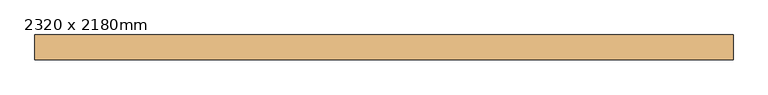
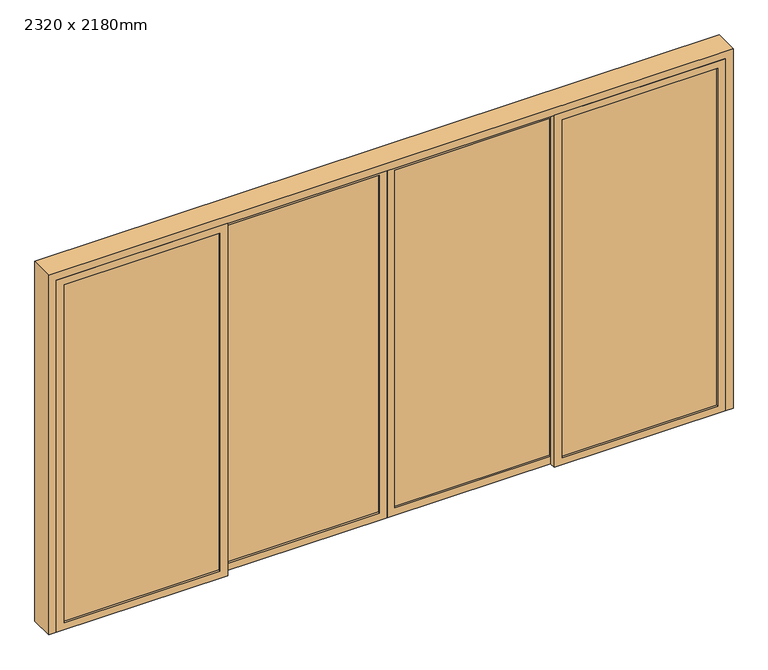
"""IFC4 building model written with IfcOpenShell, lengths in millimetres: door geometry, Porta envidraçada de correr quádrupla sem revestimento : 2320 x 2180mm."""

import ifcopenshell
import ifcopenshell.guid

model = None  # the IFC model being written
_history = None  # IfcOwnerHistory: only IFC2X3 demands one
_inside = {}  # id of a spatial element -> (the spatial element, [elements in it])
_under = {}  # id of a project, library or spatial element -> (it, [spatial elements below it])
_declared = {}  # id of a project -> (the project, [libraries it declares])
_typed = {}  # id of a type object -> (the type object, [elements of that type])
_made_of = {}  # id of a material, layer set ... -> (it, [elements and type objects made of it])


def new_model(schema):
    """Start an empty IFC model of exactly this schema.

    Asked for "IFC4X3", IfcOpenShell would pick the latest addendum, in which some entities
    have other attributes; the version numbers below select the first issue.
    IFC2X3 requires an IfcOwnerHistory on every rooted entity: one is made here for all.
    """
    global model, _history
    if schema == "IFC4X3":
        model = ifcopenshell.file(schema_version=(4, 3, 0, 0))
    else:
        model = ifcopenshell.file(schema=schema)
    _inside.clear()
    _under.clear()
    _declared.clear()
    _typed.clear()
    _made_of.clear()
    _history = None
    if model.schema == "IFC2X3":
        org = make("IfcOrganization", Name="unknown")
        user = make(
            "IfcPersonAndOrganization",
            ThePerson=make("IfcPerson", FamilyName="unknown"),
            TheOrganization=org,
        )
        app = make(
            "IfcApplication",
            ApplicationDeveloper=org,
            Version="unknown",
            ApplicationFullName="unknown",
            ApplicationIdentifier="unknown",
        )
        _history = make(
            "IfcOwnerHistory",
            OwningUser=user,
            OwningApplication=app,
            ChangeAction="ADDED",
            CreationDate=0,
        )
    return model


def make(cls, **values):
    """One entity of the class cls with the attributes given. An attribute that is None is left unset."""
    return model.create_entity(
        cls, **{name: value for name, value in values.items() if value is not None}
    )


def rooted(cls, **values):
    """An entity with a GlobalId (a new one), such as an element, a storey or a relation."""
    return make(cls, GlobalId=ifcopenshell.guid.new(), OwnerHistory=_history, **values)


def si_unit(unit_type, name, prefix=None):
    """IfcSIUnit, for example si_unit("LENGTHUNIT", "METRE", prefix="MILLI")."""
    return make("IfcSIUnit", UnitType=unit_type, Prefix=prefix, Name=name)


def assignment(units):
    """IfcUnitAssignment: the units of a project."""
    return None if units is None else make("IfcUnitAssignment", Units=units)


def point(xyz):
    """IfcCartesianPoint."""
    return None if xyz is None else make("IfcCartesianPoint", Coordinates=xyz)


def direction(xyz):
    """IfcDirection."""
    return None if xyz is None else make("IfcDirection", DirectionRatios=xyz)


def frame(location, z_axis=None, x_axis=None):
    """IfcAxis2Placement3D, a coordinate frame: its origin and axes. An axis left out is left unset."""
    return make(
        "IfcAxis2Placement3D",
        Location=point(location),
        Axis=direction(z_axis),
        RefDirection=direction(x_axis),
    )


def frame_2d(location, x_axis=None):
    """IfcAxis2Placement2D, a coordinate frame in the plane: its origin and x axis."""
    return make(
        "IfcAxis2Placement2D", Location=point(location), RefDirection=direction(x_axis)
    )


def origin():
    """The frame at (0, 0, 0) with its axes left unset."""
    return frame((0.0, 0.0, 0.0))


def place(relative_to, where):
    """IfcLocalPlacement: puts the frame where relative to a parent placement (None: the world)."""
    return make(
        "IfcLocalPlacement", PlacementRelTo=relative_to, RelativePlacement=where
    )


def context(
    kind, dimensions, precision=None, world=None, true_north=None, identifier=None
):
    """IfcGeometricRepresentationContext, for example the 3D "Model" context."""
    return make(
        "IfcGeometricRepresentationContext",
        ContextIdentifier=identifier,
        ContextType=kind,
        CoordinateSpaceDimension=dimensions,
        Precision=precision,
        WorldCoordinateSystem=world,
        TrueNorth=true_north,
    )


def project(units=None, contexts=None):
    """IfcProject with its units and contexts."""
    return rooted(
        "IfcProject",
        Name="project",
        RepresentationContexts=contexts,
        UnitsInContext=assignment(units),
    )


def spatial(cls, under=None, at=None, **own):
    """A site, building, storey or space (cls), placed at a placement, below another one or the project."""
    s = rooted(cls, ObjectPlacement=at, **own)
    if under is not None:
        _under.setdefault(under.id(), (under, []))[1].append(s)
    return s


def polyline(points):
    """IfcPolyline through the points."""
    return make("IfcPolyline", Points=[point(p) for p in points])


def circle_curve(where, radius):
    """IfcCircle in the frame where."""
    return make("IfcCircle", Position=where, Radius=radius)


def trimmed(basis, trim1, trim2, sense, master):
    """IfcTrimmedCurve: the piece of a basis curve between two trims."""
    return make(
        "IfcTrimmedCurve",
        BasisCurve=basis,
        Trim1=trim1,
        Trim2=trim2,
        SenseAgreement=sense,
        MasterRepresentation=master,
    )


def segment(curve, same_sense, transition):
    """IfcCompositeCurveSegment."""
    return make(
        "IfcCompositeCurveSegment",
        Transition=transition,
        SameSense=same_sense,
        ParentCurve=curve,
    )


def composite_curve(segments, self_intersect=None):
    """IfcCompositeCurve: segments joined end to end."""
    return make("IfcCompositeCurve", Segments=segments, SelfIntersect=self_intersect)


def outline(outer, holes=None, kind="AREA"):
    """IfcArbitraryClosedProfileDef: a profile drawn as a closed curve; with holes, ...WithVoids."""
    if holes is None:
        return make("IfcArbitraryClosedProfileDef", ProfileType=kind, OuterCurve=outer)
    return make(
        "IfcArbitraryProfileDefWithVoids",
        ProfileType=kind,
        OuterCurve=outer,
        InnerCurves=holes,
    )


def extrude(swept, where, along, depth):
    """IfcExtrudedAreaSolid: the profile swept, set in the frame where, extruded along a direction by depth."""
    return make(
        "IfcExtrudedAreaSolid",
        SweptArea=swept,
        Position=where,
        ExtrudedDirection=direction(along),
        Depth=depth,
    )


def shape(context_of_items, identifier, shape_type, items):
    """IfcShapeRepresentation: the items that make up one representation, for example the "Body"."""
    return make(
        "IfcShapeRepresentation",
        ContextOfItems=context_of_items,
        RepresentationIdentifier=identifier,
        RepresentationType=shape_type,
        Items=items,
    )


def source(mapping_origin, context_of_items, identifier, shape_type, items):
    """IfcRepresentationMap: a shape defined once, which mapped items show again and again."""
    return make(
        "IfcRepresentationMap",
        MappingOrigin=mapping_origin,
        MappedRepresentation=shape(context_of_items, identifier, shape_type, items),
    )


def transform(
    local_origin,
    x_axis=None,
    y_axis=None,
    z_axis=None,
    scale=None,
    scale2=None,
    scale3=None,
    uniform=True,
):
    """IfcCartesianTransformationOperator3D, or its non-uniform kind. x_axis, y_axis, z_axis: its Axis1, 2, 3."""
    if uniform:
        return make(
            "IfcCartesianTransformationOperator3D",
            Axis1=direction(x_axis),
            Axis2=direction(y_axis),
            LocalOrigin=point(local_origin),
            Scale=scale,
            Axis3=direction(z_axis),
        )
    return make(
        "IfcCartesianTransformationOperator3DnonUniform",
        Axis1=direction(x_axis),
        Axis2=direction(y_axis),
        LocalOrigin=point(local_origin),
        Scale=scale,
        Axis3=direction(z_axis),
        Scale2=scale2,
        Scale3=scale3,
    )


def mapped(mapping_source, mapping_target):
    """IfcMappedItem: shows the shape of a source again, moved by a transform."""
    return make(
        "IfcMappedItem", MappingSource=mapping_source, MappingTarget=mapping_target
    )


def made_of(thing, what):
    """Note that an element or type object is made of a material, layer set ...; save() writes the relation."""
    if what is not None:
        _made_of.setdefault(what.id(), (what, []))[1].append(thing)
    return thing


def element(
    cls,
    number,
    at=None,
    inside=None,
    cuts=None,
    type_object=None,
    material=None,
    context=None,
    identifier="Body",
    shape_type=None,
    held_by="IfcProductDefinitionShape",
    body=None,
    shapes=None,
    **own,
):
    """One element of the class cls, such as IfcWall. Its Tag is "e" and its number.

    at: its placement. inside: the storey or other place that contains it. cuts: it is an
    opening in that element (IfcRelVoidsElement). A single representation is given by context,
    identifier, shape_type and body (its items); several are given by shapes. held_by: the class
    of the entity that holds the representations. save() writes the other relations.
    """
    e = rooted(cls, Tag="e%d" % number, ObjectPlacement=at, **own)
    if body is not None:
        shapes = [shape(context, identifier, shape_type, body)]
    if shapes is not None:
        e.Representation = make(held_by, Representations=shapes)
    if inside is not None:
        _inside.setdefault(inside.id(), (inside, []))[1].append(e)
    if cuts is not None:
        rooted(
            "IfcRelVoidsElement", RelatingBuildingElement=cuts, RelatedOpeningElement=e
        )
    if type_object is not None:
        _typed.setdefault(type_object.id(), (type_object, []))[1].append(e)
    return made_of(e, material)


def aggregate(whole, parts):
    """IfcRelAggregates: a whole, such as a stair, and the parts it consists of."""
    return rooted("IfcRelAggregates", RelatingObject=whole, RelatedObjects=parts)


def save(model, path):
    """Write the relations noted so far, then the file.

    IfcRelAggregates (storeys below a building ...), IfcRelContainedInSpatialStructure (elements
    in a storey), IfcRelDefinesByType, IfcRelAssociatesMaterial and IfcRelDeclares: one each for
    every whole, place, type object, material and project.
    """
    for whole, parts in _under.values():
        aggregate(whole, parts)
    for where, things in _inside.values():
        rooted(
            "IfcRelContainedInSpatialStructure",
            RelatedElements=things,
            RelatingStructure=where,
        )
    for kind, things in _typed.values():
        rooted("IfcRelDefinesByType", RelatedObjects=things, RelatingType=kind)
    for what, things in _made_of.values():
        rooted("IfcRelAssociatesMaterial", RelatedObjects=things, RelatingMaterial=what)
    for by, libraries in _declared.values():
        rooted("IfcRelDeclares", RelatingContext=by, RelatedDefinitions=libraries)
    model.write(path)


def door_2320_x_2180mm_da102013(model_context):
    return source(origin(), model_context, "Body", "SweptSolid", [
        extrude(outline(composite_curve([segment(trimmed(circle_curve(frame_2d((990.0, 15.0)), 10.0), [point((1000.0, 15.0))], [point((990.0, 5.0))], False, "CARTESIAN"), True, "CONTINUOUS"), segment(polyline([(990.0, 5.0), (810.0, 5.0)]), True, "CONTINUOUS"), segment(trimmed(circle_curve(frame_2d((810.0, 15.0)), 10.0), [point((810.0, 5.0))], [point((800.0, 15.0))], False, "CARTESIAN"), True, "CONTINUOUS"), segment(polyline([(800.0, 15.0), (800.0, 35.0)]), True, "CONTINUOUS"), segment(trimmed(circle_curve(frame_2d((810.0, 35.0)), 10.0), [point((800.0, 35.0))], [point((810.0, 45.0))], False, "CARTESIAN"), True, "CONTINUOUS"), segment(polyline([(810.0, 45.0), (990.0, 45.0)]), True, "CONTINUOUS"), segment(trimmed(circle_curve(frame_2d((990.0, 35.0)), 10.0), [point((990.0, 45.0))], [point((1000.0, 35.0))], False, "CARTESIAN"), True, "CONTINUOUS"), segment(polyline([(1000.0, 35.0), (1000.0, 15.0)]), True, "CONTINUOUS")], self_intersect=False), holes=[composite_curve([segment(trimmed(circle_curve(frame_2d((985.0, 25.0)), 5.0), [point((985.0, 20.0))], [point((985.0, 30.0))], True, "CARTESIAN"), True, "CONTINUOUS"), segment(trimmed(circle_curve(frame_2d((985.0, 25.0)), 5.0), [point((985.0, 30.0))], [point((985.0, 20.0))], True, "CARTESIAN"), True, "CONTINUOUS")], self_intersect=False), composite_curve([segment(trimmed(circle_curve(frame_2d((815.0, 25.0)), 5.0), [point((815.0, 20.0))], [point((815.0, 30.0))], True, "CARTESIAN"), True, "CONTINUOUS"), segment(trimmed(circle_curve(frame_2d((815.0, 25.0)), 5.0), [point((815.0, 30.0))], [point((815.0, 20.0))], True, "CARTESIAN"), True, "CONTINUOUS")], self_intersect=False), composite_curve([segment(polyline([(960.0, 15.0), (960.0, 35.0)]), True, "CONTINUOUS"), segment(trimmed(circle_curve(frame_2d((955.0, 35.0)), 5.0), [point((960.0, 35.0))], [point((955.0, 40.0))], True, "CARTESIAN"), True, "CONTINUOUS"), segment(polyline([(955.0, 40.0), (845.0, 40.0)]), True, "CONTINUOUS"), segment(trimmed(circle_curve(frame_2d((845.0, 35.0)), 5.0), [point((845.0, 40.0))], [point((840.0, 35.0))], True, "CARTESIAN"), True, "CONTINUOUS"), segment(polyline([(840.0, 35.0), (840.0, 15.0)]), True, "CONTINUOUS"), segment(trimmed(circle_curve(frame_2d((845.0, 15.0)), 5.0), [point((840.0, 15.0))], [point((845.0, 10.0))], True, "CARTESIAN"), True, "CONTINUOUS"), segment(polyline([(845.0, 10.0), (955.0, 10.0)]), True, "CONTINUOUS"), segment(trimmed(circle_curve(frame_2d((955.0, 15.0)), 5.0), [point((955.0, 10.0))], [point((960.0, 15.0))], True, "CARTESIAN"), True, "CONTINUOUS")], self_intersect=False)]), frame((0.0, 5.4, 0.0), z_axis=(0.0, 1.0, 0.0), x_axis=(0.0, 0.0, 1.0)), (0.0, 0.0, 1.0), 3.0),
        extrude(outline(composite_curve([segment(trimmed(circle_curve(frame_2d((990.0, -35.0)), 10.0), [point((1000.0, -35.0))], [point((990.0, -45.0))], False, "CARTESIAN"), True, "CONTINUOUS"), segment(polyline([(990.0, -45.0), (810.0, -45.0)]), True, "CONTINUOUS"), segment(trimmed(circle_curve(frame_2d((810.0, -35.0)), 10.0), [point((810.0, -45.0))], [point((800.0, -35.0))], False, "CARTESIAN"), True, "CONTINUOUS"), segment(polyline([(800.0, -35.0), (800.0, -15.0)]), True, "CONTINUOUS"), segment(trimmed(circle_curve(frame_2d((810.0, -15.0)), 10.0), [point((800.0, -15.0))], [point((810.0, -5.0))], False, "CARTESIAN"), True, "CONTINUOUS"), segment(polyline([(810.0, -5.0), (990.0, -5.0)]), True, "CONTINUOUS"), segment(trimmed(circle_curve(frame_2d((990.0, -15.0)), 10.0), [point((990.0, -5.0))], [point((1000.0, -15.0))], False, "CARTESIAN"), True, "CONTINUOUS"), segment(polyline([(1000.0, -15.0), (1000.0, -35.0)]), True, "CONTINUOUS")], self_intersect=False), holes=[composite_curve([segment(trimmed(circle_curve(frame_2d((985.0, -25.0)), 5.0), [point((985.0, -30.0))], [point((985.0, -20.0))], True, "CARTESIAN"), True, "CONTINUOUS"), segment(trimmed(circle_curve(frame_2d((985.0, -25.0)), 5.0), [point((985.0, -20.0))], [point((985.0, -30.0))], True, "CARTESIAN"), True, "CONTINUOUS")], self_intersect=False), composite_curve([segment(trimmed(circle_curve(frame_2d((815.0, -25.0)), 5.0), [point((815.0, -30.0))], [point((815.0, -20.0))], True, "CARTESIAN"), True, "CONTINUOUS"), segment(trimmed(circle_curve(frame_2d((815.0, -25.0)), 5.0), [point((815.0, -20.0))], [point((815.0, -30.0))], True, "CARTESIAN"), True, "CONTINUOUS")], self_intersect=False), composite_curve([segment(polyline([(960.0, -35.0), (960.0, -15.0)]), True, "CONTINUOUS"), segment(trimmed(circle_curve(frame_2d((955.0, -15.0)), 5.0), [point((960.0, -15.0))], [point((955.0, -10.0))], True, "CARTESIAN"), True, "CONTINUOUS"), segment(polyline([(955.0, -10.0), (845.0, -10.0)]), True, "CONTINUOUS"), segment(trimmed(circle_curve(frame_2d((845.0, -15.0)), 5.0), [point((845.0, -10.0))], [point((840.0, -15.0))], True, "CARTESIAN"), True, "CONTINUOUS"), segment(polyline([(840.0, -15.0), (840.0, -35.0)]), True, "CONTINUOUS"), segment(trimmed(circle_curve(frame_2d((845.0, -35.0)), 5.0), [point((840.0, -35.0))], [point((845.0, -40.0))], True, "CARTESIAN"), True, "CONTINUOUS"), segment(polyline([(845.0, -40.0), (955.0, -40.0)]), True, "CONTINUOUS"), segment(trimmed(circle_curve(frame_2d((955.0, -35.0)), 5.0), [point((955.0, -40.0))], [point((960.0, -35.0))], True, "CARTESIAN"), True, "CONTINUOUS")], self_intersect=False)]), frame((0.0, 5.4, 0.0), z_axis=(0.0, 1.0, 0.0), x_axis=(0.0, 0.0, 1.0)), (0.0, 0.0, 1.0), 3.0),
        extrude(outline(polyline([(2450.0, -1125.0), (0.0, -1125.0), (0.0, 0.0), (2450.0, 0.0), (2450.0, -1125.0)]), holes=[polyline([(2400.0, -50.0), (50.0, -50.0), (50.0, -1075.0), (2400.0, -1075.0), (2400.0, -50.0)])]), frame((0.0, -34.6, 0.0), z_axis=(0.0, 1.0, 0.0), x_axis=(0.0, 0.0, 1.0)), (0.0, 0.0, 1.0), 40.0),
        extrude(outline(polyline([(2450.0, 1075.0), (0.0, 1075.0), (0.0, 2200.0), (2450.0, 2200.0), (2450.0, 1075.0)]), holes=[polyline([(2400.0, 2150.0), (50.0, 2150.0), (50.0, 1125.0), (2400.0, 1125.0), (2400.0, 2150.0)])]), frame((0.0, -79.6, 0.0), z_axis=(0.0, 1.0, 0.0), x_axis=(0.0, 0.0, 1.0)), (0.0, 0.0, 1.0), 40.0),
        extrude(outline(polyline([(2450.0, 0.0), (0.0, 0.0), (0.0, 1125.0), (2450.0, 1125.0), (2450.0, 0.0)]), holes=[polyline([(2400.0, 1075.0), (50.0, 1075.0), (50.0, 50.0), (2400.0, 50.0), (2400.0, 1075.0)])]), frame((0.0, -34.6, 0.0), z_axis=(0.0, 1.0, 0.0), x_axis=(0.0, 0.0, 1.0)), (0.0, 0.0, 1.0), 40.0),
        extrude(outline(polyline([(2450.0, -2200.0), (0.0, -2200.0), (0.0, -1075.0), (2450.0, -1075.0), (2450.0, -2200.0)]), holes=[polyline([(2400.0, -1125.0), (50.0, -1125.0), (50.0, -2150.0), (2400.0, -2150.0), (2400.0, -1125.0)])]), frame((0.0, -79.6, 0.0), z_axis=(0.0, 1.0, 0.0), x_axis=(0.0, 0.0, 1.0)), (0.0, 0.0, 1.0), 40.0),
        extrude(outline(polyline([(0.0, 2200.0), (0.0, 2250.0), (2500.0, 2250.0), (2500.0, -2250.0), (0.0, -2250.0), (0.0, -2200.0), (2450.0, -2200.0), (2450.0, 2200.0), (0.0, 2200.0)])), frame((0.0, -79.6, 0.0), z_axis=(0.0, 1.0, 0.0), x_axis=(0.0, 0.0, 1.0)), (0.0, 0.0, 1.0), 159.2),
        extrude(outline(polyline([(1075.0, -7.6), (1075.0, -21.6), (50.0, -21.6), (50.0, -7.6), (1075.0, -7.6)])), frame((0.0, 0.0, 50.0), z_axis=(0.0, 0.0, 1.0), x_axis=(1.0, 0.0, 0.0)), (0.0, 0.0, 1.0), 2350.0),
        extrude(outline(polyline([(2150.0, -52.6), (2150.0, -66.6), (1125.0, -66.6), (1125.0, -52.6), (2150.0, -52.6)])), frame((0.0, 0.0, 50.0), z_axis=(0.0, 0.0, 1.0), x_axis=(1.0, 0.0, 0.0)), (0.0, 0.0, 1.0), 2350.0),
        extrude(outline(polyline([(-1125.0, -52.6), (-1125.0, -66.6), (-2150.0, -66.6), (-2150.0, -52.6), (-1125.0, -52.6)])), frame((0.0, 0.0, 50.0), z_axis=(0.0, 0.0, 1.0), x_axis=(1.0, 0.0, 0.0)), (0.0, 0.0, 1.0), 2350.0),
        extrude(outline(polyline([(-50.0, -7.6), (-50.0, -21.6), (-1075.0, -21.6), (-1075.0, -7.6), (-50.0, -7.6)])), frame((0.0, 0.0, 50.0), z_axis=(0.0, 0.0, 1.0), x_axis=(1.0, 0.0, 0.0)), (0.0, 0.0, 1.0), 2350.0),
        extrude(outline(polyline([(-1125.0, -52.6), (-1125.0, -66.6), (-2150.0, -66.6), (-2150.0, -52.6), (-1125.0, -52.6)])), frame((0.0, 0.0, 50.0), z_axis=(0.0, 0.0, 1.0), x_axis=(1.0, 0.0, 0.0)), (0.0, 0.0, 1.0), 2350.0),
        extrude(outline(polyline([(-50.0, -7.6), (-50.0, -21.6), (-1075.0, -21.6), (-1075.0, -7.6), (-50.0, -7.6)])), frame((0.0, 0.0, 50.0), z_axis=(0.0, 0.0, 1.0), x_axis=(1.0, 0.0, 0.0)), (0.0, 0.0, 1.0), 2350.0),
        extrude(outline(polyline([(1125.0, -52.6), (2150.0, -52.6), (2150.0, -66.6), (1125.0, -66.6), (1125.0, -52.6)])), frame((0.0, 0.0, 50.0), z_axis=(0.0, 0.0, 1.0), x_axis=(1.0, 0.0, 0.0)), (0.0, 0.0, 1.0), 2350.0),
        extrude(outline(polyline([(50.0, -7.6), (1075.0, -7.6), (1075.0, -21.6), (50.0, -21.6), (50.0, -7.6)])), frame((0.0, 0.0, 50.0), z_axis=(0.0, 0.0, 1.0), x_axis=(1.0, 0.0, 0.0)), (0.0, 0.0, 1.0), 2350.0),
    ])


if __name__ == "__main__":
    model = new_model("IFC4")
    model_context = context("Model", 3, world=origin())
    ifc_project = project(units=[si_unit("LENGTHUNIT", "METRE", prefix="MILLI")], contexts=[model_context])
    site = spatial("IfcSite", under=ifc_project)
    building = spatial("IfcBuilding", under=site)
    placement = place(None, origin())
    door_2320_x_2180mm_shape = door_2320_x_2180mm_da102013(model_context)
    element("IfcDoor", 1, ObjectType="Porta envidraçada de correr quádrupla sem revestimento : 2320 x 2180mm", at=placement, inside=building, context=model_context, shape_type="MappedRepresentation", body=[
        mapped(door_2320_x_2180mm_shape, transform((0.0, 0.0, 0.0), x_axis=(1.0, 0.0, 0.0), y_axis=(0.0, 1.0, 0.0), z_axis=(0.0, 0.0, 1.0))),
    ])
    save(model, "model.ifc")

# Revit data of these elements
# Type "Porta envidraçada de correr quádrupla sem revestimento : 2320 x 2180mm"
#   Type Mark = "P50"
#   Construction Type Id = "GSP4R"
#   Analytic Construction = "Vidraça única Pilkington 1/8 pol"
#   Visual Light Transmittance = 0.9
#   Solar Heat Gain Coefficient = 0.78
#   Rough Width = 4.50 m
#   Rough Height = 2.50 m
#   Largura da moldura do painel = 0.05 m
#   Espessura da moldura do painel = 0.04 m
#   Heat Transfer Coefficient (U) = 3.6886 W/(m²·K)
#   Largura da maçaneta = 0.04 m
#   Altura do puxador = 0.20 m
#   Largura da estrutura = 0.05 m
#   Height = 2.50 m
#   Width = 4.50 m
#   Function = 1
#   Material do puxador = none
#   Vidro = Vidro - Janela
#   Material da estrutura = Aluminum Sill
#   Thickness = 0
#   Wall Closure = (empty or 0)
# Element 1 (IfcDoor, "Porta envidraçada de correr quádrupla sem revestimento : 2320 x 2180mm")
#   Materials on its faces: "Aluminum Sill", "Vidro - Janela"
# Materials
#   "Vidro - Janela": class "Vidro", colour RGB 249 249 249, transparency 1, Cost = 0
#   "Aluminum Sill": class "Não atribuído", colour RGB 247 247 247, transparency 0
